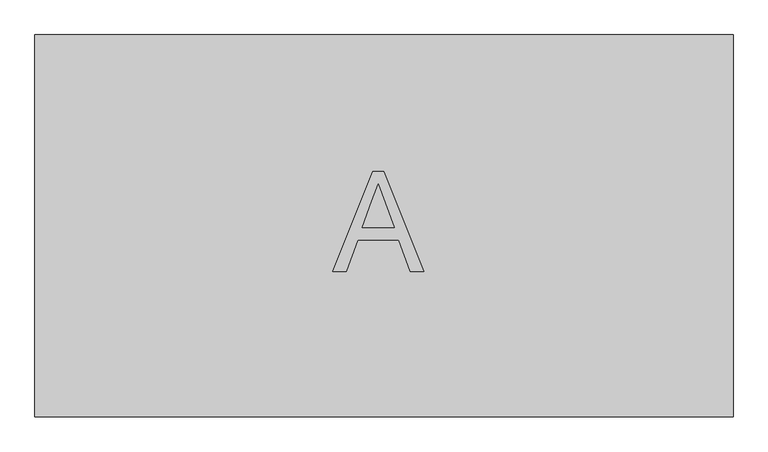
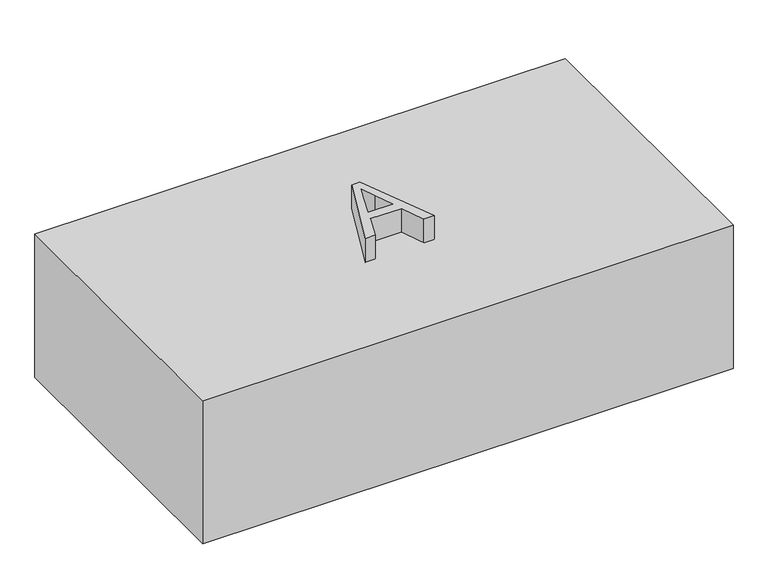
"""IFC4 building model written with IfcOpenShell, lengths in millimetres: proxy geometry, The Messy Family A : The Messy Family A."""

from ifc_helpers import new_model, si_unit, frame, origin, origin_with_axes, place, context, project, spatial, polyline, outline, extrude, source, transform, mapped, element, save


def generic_models_50cfcde5(model_context):
    return source(origin(), model_context, "Body", "SweptSolid", [
        extrude(outline(polyline([(541.9415527, 284.565081), (541.9415527, -299.634919), (-524.8584473, -299.634919), (-524.8584473, 284.565081), (541.9415527, 284.565081)])), origin_with_axes(), (0.0, 0.0, 1.0), 304.8),
        extrude(outline(polyline([(-69.5890348, -77.2556777), (-8.4779493, 75.839739), (7.8183402, 75.839739), (68.9294257, -77.2556777), (48.7085711, -77.2556777), (31.1788469, -29.41336), (-31.8758328, -29.41336), (-49.3681802, -77.2556777), (-69.5890348, -77.2556777)]), holes=[polyline([(-24.8489924, -10.2764329), (24.1893833, -10.2764329), (10.3973401, 27.3620155), (-0.3298045, 56.7028119), (-9.8608913, 30.6511748), (-24.8489924, -10.2764329)])]), frame((0.0, 0.0, 304.8), z_axis=(0.0, 0.0, 1.0), x_axis=(1.0, 0.0, 0.0)), (0.0, 0.0, 1.0), 50.8),
    ])


if __name__ == "__main__":
    model = new_model("IFC4")
    model_context = context("Model", 3, world=origin())
    ifc_project = project(units=[si_unit("LENGTHUNIT", "METRE", prefix="MILLI")], contexts=[model_context])
    site = spatial("IfcSite", under=ifc_project)
    building = spatial("IfcBuilding", under=site)
    placement = place(None, origin())
    generic_models_shape = generic_models_50cfcde5(model_context)
    element("IfcBuildingElementProxy", 1, Name="The Messy Family A : The Messy Family A", ObjectType="The Messy Family A : The Messy Family A", at=placement, inside=building, context=model_context, shape_type="MappedRepresentation", body=[
        mapped(generic_models_shape, transform((0.0, 0.0, 0.0), x_axis=(1.0, 0.0, 0.0), y_axis=(0.0, 1.0, 0.0), z_axis=(0.0, 0.0, 1.0))),
    ])
    save(model, "model.ifc")

# Revit data of these elements
# Type "The Messy Family A : The Messy Family A"
#   TBC-Parameter 2 = ""
#   TBC-Parameter 1 = ""
#   Other Company Parameter 2 = ""
#   Other Company Parameter 1 = ""
#   TBC-Parameter 3 = 2' - 0"
#   Other Company Parameter 3 = 1' - 0"
#   Default Elevation = 0
